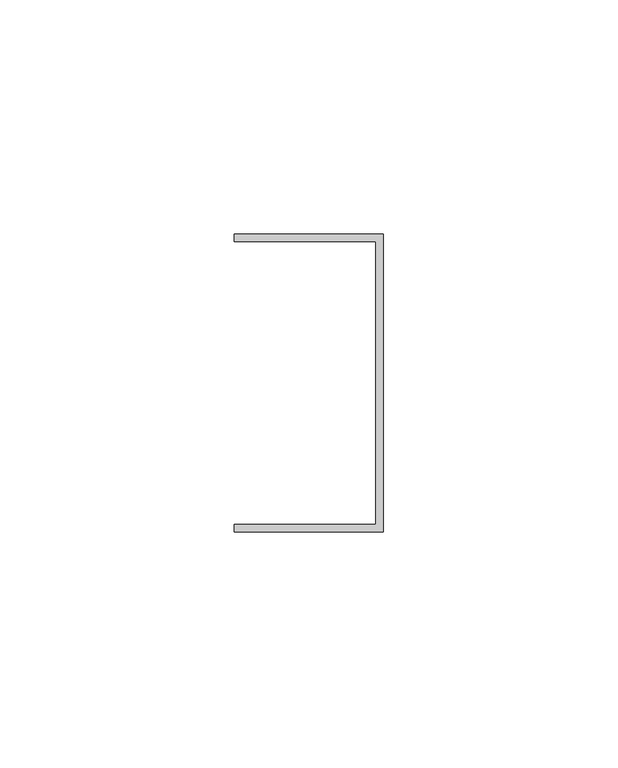
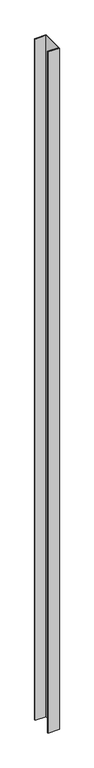
"""IFC4 building model written with IfcOpenShell, lengths in millimetres: proxy geometry, Generic Models 7:Generic Models 1:3:Generic Models 1:3 : Generic Models 7:Generic Models 1:305549:3:Generic Models 1:3:Generic Models 1:3 : Generic Models 7:Generic Models 1:305549:3 : Generic Models 7:Generic Models 1:3:Generic Models 1:3 : Generic Models 7:Generic Models 1:305549:301244:13 : Generic Models 7:Generic Models 1:3:Generic Models 1:3 : Generic Models 7:Generic Models 1:305549:3:Generic Models 1:3:Generic Models 1:3 : Generic Models 7:Generic Models 1:305549:3 : Generic Models 7:Generic Models 1:3:Generic Models 1:3 : Generic Models 7:Generic Models 1:305549:301244:308848."""

from ifc_helpers import new_model, si_unit, frame, origin, place, context, project, spatial, polyline, outline, extrude, source, transform, mapped, element, save


def generic_models_f9c75a09(model_context):
    return source(origin(), model_context, "Body", "SweptSolid", [
        extrude(outline(polyline([(578895.7226038, -579013.3913842), (578895.7226038, -579076.891384), (578863.9726038, -579076.891384), (578863.9726038, -579075.303884), (578894.1351038, -579075.303884), (578894.1351038, -579014.9788842), (578863.9726038, -579014.9788842), (578863.9726038, -579013.3913842), (578895.7226038, -579013.3913842)])), frame((0.0, 0.0, 4133.81326), z_axis=(0.0, 0.0, 1.0), x_axis=(1.0, 0.0, 0.0)), (0.0, 0.0, 1.0), 2000.28674),
    ])


if __name__ == "__main__":
    model = new_model("IFC4")
    model_context = context("Model", 3, world=origin())
    ifc_project = project(units=[si_unit("LENGTHUNIT", "METRE", prefix="MILLI")], contexts=[model_context])
    site = spatial("IfcSite", under=ifc_project)
    building = spatial("IfcBuilding", under=site)
    placement = place(None, origin())
    generic_models_shape = generic_models_f9c75a09(model_context)
    element("IfcBuildingElementProxy", 1, Name="Generic Models 7:Generic Models 1:3:Generic Models 1:3 : Generic Models 7:Generic Models 1:305549:3:Generic Models 1:3:Generic Models 1:3 : Generic Models 7:Generic Models 1:305549:3 : Generic Models 7:Generic Models 1:3:Generic Models 1:3 : Generic Models 7:Generic Models 1:305549:301244:13 : Generic Models 7:Generic Models 1:3:Generic Models 1:3 : Generic Models 7:Generic Models 1:305549:3:Generic Models 1:3:Generic Models 1:3 : Generic Models 7:Generic Models 1:305549:3 : Generic Models 7:Generic Models 1:3:Generic Models 1:3 : Generic Models 7:Generic Models 1:305549:301244:308848", ObjectType="Generic Models 7:Generic Models 1:3:Generic Models 1:3 : Generic Models 7:Generic Models 1:305549:3:Generic Models 1:3:Generic Models 1:3 : Generic Models 7:Generic Models 1:305549:3 : Generic Models 7:Generic Models 1:3:Generic Models 1:3 : Generic Models 7:Generic Models 1:305549:301244:13 : Generic Models 7:Generic Models 1:3:Generic Models 1:3 : Generic Models 7:Generic Models 1:305549:3:Generic Models 1:3:Generic Models 1:3 : Generic Models 7:Generic Models 1:305549:3 : Generic Models 7:Generic Models 1:3:Generic Models 1:3 : Generic Models 7:Generic Models 1:305549:301244:308848", at=placement, inside=building, context=model_context, shape_type="MappedRepresentation", body=[
        mapped(generic_models_shape, transform((0.0, 0.0, 0.0), x_axis=(1.0, 0.0, 0.0), y_axis=(0.0, 1.0, 0.0), z_axis=(0.0, 0.0, 1.0))),
    ])
    save(model, "model.ifc")

# Revit data of these elements
# Type "Generic Models 7:Generic Models 1:3:Generic Models 1:3 : Generic Models 7:Generic Models 1:305549:3:Generic Models 1:3:Generic Models 1:3 : Generic Models 7:Generic Models 1:305549:3 : Generic Models 7:Generic Models 1:3:Generic Models 1:3 : Generic Models 7:Generic Models 1:305549:301244:13 : Generic Models 7:Generic Models 1:3:Generic Models 1:3 : Generic Models 7:Generic Models 1:305549:3:Generic Models 1:3:Generic Models 1:3 : Generic Models 7:Generic Models 1:305549:3 : Generic Models 7:Generic Models 1:3:Generic Models 1:3 : Generic Models 7:Generic Models 1:305549:301244:308848"
#   NameOverride = "Generic Models 7:Generic Models 1:3:Generic Models 1:3 : Generic Models 7:Generic Models 1:305549:3:Generic Models 1:3:Generic Models 1:3 : Generic Models 7:Generic Models 1:305549:3 : Generic Models 7:Generic Models 1:3:Generic Models 1:3 : Generic Models 7:Generic Models 1:305549:301244:308848"
#   ObjectTypeOverride = "Generic Models 1:3:Generic Models 1:3 : Generic Models 7:Generic Models 1:305549:3 : Generic Models 7:Generic Models 1:3:Generic Models 1:3 : Generic Models 7:Generic Models 1:305549:301244"
#   Reference = "Generic Models 1"
#   Tag = "308848"
# Element 1 (IfcBuildingElementProxy, "Generic Models 7:Generic Models 1:3:Generic Models 1:3 : Generic Models 7:Generic Models 1:305549:3:Generic Models 1:3:Generic Models 1:3 : Generic Models 7:Generic Models 1:305549:3 : Generic Models 7:Generic Models 1:3:Generic Models 1:3 : Generic Models 7:Generic Models 1:305549:301244:13 : Generic Models 7:Generic Models 1:3:Generic Models 1:3 : Generic Models 7:Generic Models 1:305549:3:Generic Models 1:3:Generic Models 1:3 : Generic Models 7:Generic Models 1:305549:3 : Generic Models 7:Generic Models 1:3:Generic Models 1:3 : Generic Models 7:Generic Models 1:305549:301244:308848")
#   Materials on its faces: "GALVANIZED U-CHANNEL (250T125-33)"
# Materials
#   "GALVANIZED U-CHANNEL (250T125-33)": class "Unassigned", colour RGB 202 201 200, transparency 0, Keynote = "M05451300.02", Cost = 0
